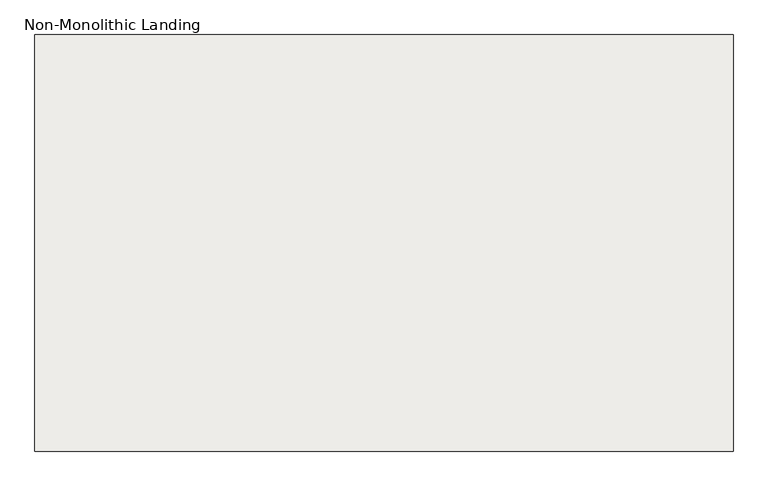
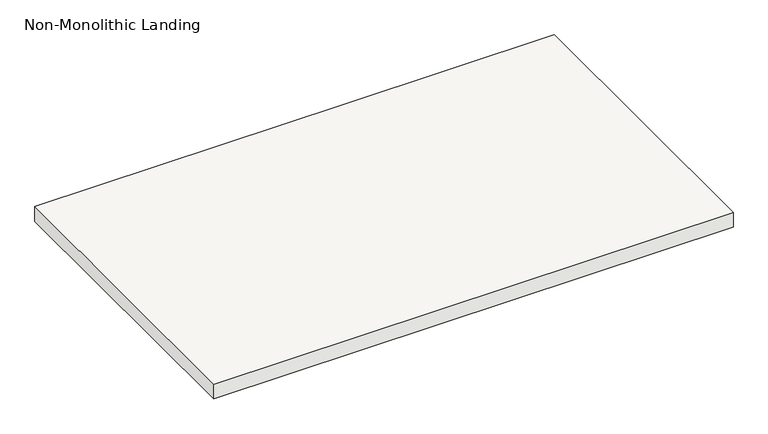
"""IFC4 building model written with IfcOpenShell, lengths in millimetres: slab geometry, Non-Monolithic Landing."""

import ifcopenshell
import ifcopenshell.guid

model = None  # the IFC model being written
_history = None  # IfcOwnerHistory: only IFC2X3 demands one
_inside = {}  # id of a spatial element -> (the spatial element, [elements in it])
_under = {}  # id of a project, library or spatial element -> (it, [spatial elements below it])
_declared = {}  # id of a project -> (the project, [libraries it declares])
_typed = {}  # id of a type object -> (the type object, [elements of that type])
_made_of = {}  # id of a material, layer set ... -> (it, [elements and type objects made of it])


def new_model(schema):
    """Start an empty IFC model of exactly this schema.

    Asked for "IFC4X3", IfcOpenShell would pick the latest addendum, in which some entities
    have other attributes; the version numbers below select the first issue.
    IFC2X3 requires an IfcOwnerHistory on every rooted entity: one is made here for all.
    """
    global model, _history
    if schema == "IFC4X3":
        model = ifcopenshell.file(schema_version=(4, 3, 0, 0))
    else:
        model = ifcopenshell.file(schema=schema)
    _inside.clear()
    _under.clear()
    _declared.clear()
    _typed.clear()
    _made_of.clear()
    _history = None
    if model.schema == "IFC2X3":
        org = make("IfcOrganization", Name="unknown")
        user = make(
            "IfcPersonAndOrganization",
            ThePerson=make("IfcPerson", FamilyName="unknown"),
            TheOrganization=org,
        )
        app = make(
            "IfcApplication",
            ApplicationDeveloper=org,
            Version="unknown",
            ApplicationFullName="unknown",
            ApplicationIdentifier="unknown",
        )
        _history = make(
            "IfcOwnerHistory",
            OwningUser=user,
            OwningApplication=app,
            ChangeAction="ADDED",
            CreationDate=0,
        )
    return model


def make(cls, **values):
    """One entity of the class cls with the attributes given. An attribute that is None is left unset."""
    return model.create_entity(
        cls, **{name: value for name, value in values.items() if value is not None}
    )


def rooted(cls, **values):
    """An entity with a GlobalId (a new one), such as an element, a storey or a relation."""
    return make(cls, GlobalId=ifcopenshell.guid.new(), OwnerHistory=_history, **values)


def si_unit(unit_type, name, prefix=None):
    """IfcSIUnit, for example si_unit("LENGTHUNIT", "METRE", prefix="MILLI")."""
    return make("IfcSIUnit", UnitType=unit_type, Prefix=prefix, Name=name)


def assignment(units):
    """IfcUnitAssignment: the units of a project."""
    return None if units is None else make("IfcUnitAssignment", Units=units)


def point(xyz):
    """IfcCartesianPoint."""
    return None if xyz is None else make("IfcCartesianPoint", Coordinates=xyz)


def direction(xyz):
    """IfcDirection."""
    return None if xyz is None else make("IfcDirection", DirectionRatios=xyz)


def frame(location, z_axis=None, x_axis=None):
    """IfcAxis2Placement3D, a coordinate frame: its origin and axes. An axis left out is left unset."""
    return make(
        "IfcAxis2Placement3D",
        Location=point(location),
        Axis=direction(z_axis),
        RefDirection=direction(x_axis),
    )


def origin():
    """The frame at (0, 0, 0) with its axes left unset."""
    return frame((0.0, 0.0, 0.0))


def place(relative_to, where):
    """IfcLocalPlacement: puts the frame where relative to a parent placement (None: the world)."""
    return make(
        "IfcLocalPlacement", PlacementRelTo=relative_to, RelativePlacement=where
    )


def context(
    kind, dimensions, precision=None, world=None, true_north=None, identifier=None
):
    """IfcGeometricRepresentationContext, for example the 3D "Model" context."""
    return make(
        "IfcGeometricRepresentationContext",
        ContextIdentifier=identifier,
        ContextType=kind,
        CoordinateSpaceDimension=dimensions,
        Precision=precision,
        WorldCoordinateSystem=world,
        TrueNorth=true_north,
    )


def project(units=None, contexts=None):
    """IfcProject with its units and contexts."""
    return rooted(
        "IfcProject",
        Name="project",
        RepresentationContexts=contexts,
        UnitsInContext=assignment(units),
    )


def spatial(cls, under=None, at=None, **own):
    """A site, building, storey or space (cls), placed at a placement, below another one or the project."""
    s = rooted(cls, ObjectPlacement=at, **own)
    if under is not None:
        _under.setdefault(under.id(), (under, []))[1].append(s)
    return s


def polyline(points):
    """IfcPolyline through the points."""
    return make("IfcPolyline", Points=[point(p) for p in points])


def outline(outer, holes=None, kind="AREA"):
    """IfcArbitraryClosedProfileDef: a profile drawn as a closed curve; with holes, ...WithVoids."""
    if holes is None:
        return make("IfcArbitraryClosedProfileDef", ProfileType=kind, OuterCurve=outer)
    return make(
        "IfcArbitraryProfileDefWithVoids",
        ProfileType=kind,
        OuterCurve=outer,
        InnerCurves=holes,
    )


def extrude(swept, where, along, depth):
    """IfcExtrudedAreaSolid: the profile swept, set in the frame where, extruded along a direction by depth."""
    return make(
        "IfcExtrudedAreaSolid",
        SweptArea=swept,
        Position=where,
        ExtrudedDirection=direction(along),
        Depth=depth,
    )


def shape(context_of_items, identifier, shape_type, items):
    """IfcShapeRepresentation: the items that make up one representation, for example the "Body"."""
    return make(
        "IfcShapeRepresentation",
        ContextOfItems=context_of_items,
        RepresentationIdentifier=identifier,
        RepresentationType=shape_type,
        Items=items,
    )


def source(mapping_origin, context_of_items, identifier, shape_type, items):
    """IfcRepresentationMap: a shape defined once, which mapped items show again and again."""
    return make(
        "IfcRepresentationMap",
        MappingOrigin=mapping_origin,
        MappedRepresentation=shape(context_of_items, identifier, shape_type, items),
    )


def transform(
    local_origin,
    x_axis=None,
    y_axis=None,
    z_axis=None,
    scale=None,
    scale2=None,
    scale3=None,
    uniform=True,
):
    """IfcCartesianTransformationOperator3D, or its non-uniform kind. x_axis, y_axis, z_axis: its Axis1, 2, 3."""
    if uniform:
        return make(
            "IfcCartesianTransformationOperator3D",
            Axis1=direction(x_axis),
            Axis2=direction(y_axis),
            LocalOrigin=point(local_origin),
            Scale=scale,
            Axis3=direction(z_axis),
        )
    return make(
        "IfcCartesianTransformationOperator3DnonUniform",
        Axis1=direction(x_axis),
        Axis2=direction(y_axis),
        LocalOrigin=point(local_origin),
        Scale=scale,
        Axis3=direction(z_axis),
        Scale2=scale2,
        Scale3=scale3,
    )


def mapped(mapping_source, mapping_target):
    """IfcMappedItem: shows the shape of a source again, moved by a transform."""
    return make(
        "IfcMappedItem", MappingSource=mapping_source, MappingTarget=mapping_target
    )


def made_of(thing, what):
    """Note that an element or type object is made of a material, layer set ...; save() writes the relation."""
    if what is not None:
        _made_of.setdefault(what.id(), (what, []))[1].append(thing)
    return thing


def element(
    cls,
    number,
    at=None,
    inside=None,
    cuts=None,
    type_object=None,
    material=None,
    context=None,
    identifier="Body",
    shape_type=None,
    held_by="IfcProductDefinitionShape",
    body=None,
    shapes=None,
    **own,
):
    """One element of the class cls, such as IfcWall. Its Tag is "e" and its number.

    at: its placement. inside: the storey or other place that contains it. cuts: it is an
    opening in that element (IfcRelVoidsElement). A single representation is given by context,
    identifier, shape_type and body (its items); several are given by shapes. held_by: the class
    of the entity that holds the representations. save() writes the other relations.
    """
    e = rooted(cls, Tag="e%d" % number, ObjectPlacement=at, **own)
    if body is not None:
        shapes = [shape(context, identifier, shape_type, body)]
    if shapes is not None:
        e.Representation = make(held_by, Representations=shapes)
    if inside is not None:
        _inside.setdefault(inside.id(), (inside, []))[1].append(e)
    if cuts is not None:
        rooted(
            "IfcRelVoidsElement", RelatingBuildingElement=cuts, RelatedOpeningElement=e
        )
    if type_object is not None:
        _typed.setdefault(type_object.id(), (type_object, []))[1].append(e)
    return made_of(e, material)


def aggregate(whole, parts):
    """IfcRelAggregates: a whole, such as a stair, and the parts it consists of."""
    return rooted("IfcRelAggregates", RelatingObject=whole, RelatedObjects=parts)


def save(model, path):
    """Write the relations noted so far, then the file.

    IfcRelAggregates (storeys below a building ...), IfcRelContainedInSpatialStructure (elements
    in a storey), IfcRelDefinesByType, IfcRelAssociatesMaterial and IfcRelDeclares: one each for
    every whole, place, type object, material and project.
    """
    for whole, parts in _under.values():
        aggregate(whole, parts)
    for where, things in _inside.values():
        rooted(
            "IfcRelContainedInSpatialStructure",
            RelatedElements=things,
            RelatingStructure=where,
        )
    for kind, things in _typed.values():
        rooted("IfcRelDefinesByType", RelatedObjects=things, RelatingType=kind)
    for what, things in _made_of.values():
        rooted("IfcRelAssociatesMaterial", RelatedObjects=things, RelatingMaterial=what)
    for by, libraries in _declared.values():
        rooted("IfcRelDeclares", RelatingContext=by, RelatedDefinitions=libraries)
    model.write(path)


def non_monolithic_landing_18e61c0d(model_context):
    return source(origin(), model_context, "Body", "SweptSolid", [
        extrude(outline(polyline([(-13281.6736899, -2171.6396273), (-12605.9172363, -2171.6396273), (-12605.9172363, -3171.6396273), (-14281.6736899, -3171.6396273), (-14281.6736899, -2171.6396273), (-13281.6736899, -2171.6396273)])), frame((0.0, 0.0, 1859.0909091), z_axis=(0.0, 0.0, 1.0), x_axis=(1.0, 0.0, 0.0)), (0.0, 0.0, 1.0), 50.0),
    ])


if __name__ == "__main__":
    model = new_model("IFC4")
    model_context = context("Model", 3, world=origin())
    ifc_project = project(units=[si_unit("LENGTHUNIT", "METRE", prefix="MILLI")], contexts=[model_context])
    site = spatial("IfcSite", under=ifc_project)
    building = spatial("IfcBuilding", under=site)
    placement = place(None, origin())
    non_monolithic_landing_shape = non_monolithic_landing_18e61c0d(model_context)
    element("IfcSlab", 1, ObjectType="Non-Monolithic Landing", at=placement, inside=building, context=model_context, shape_type="MappedRepresentation", body=[
        mapped(non_monolithic_landing_shape, transform((0.0, 0.0, 0.0), x_axis=(1.0, 0.0, 0.0), y_axis=(0.0, 1.0, 0.0), z_axis=(0.0, 0.0, 1.0))),
    ])
    save(model, "model.ifc")
